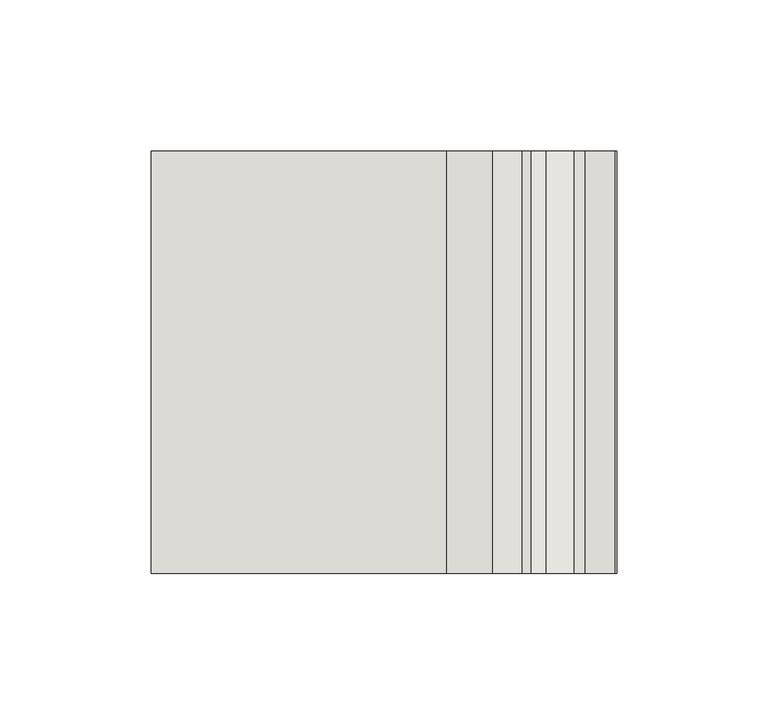
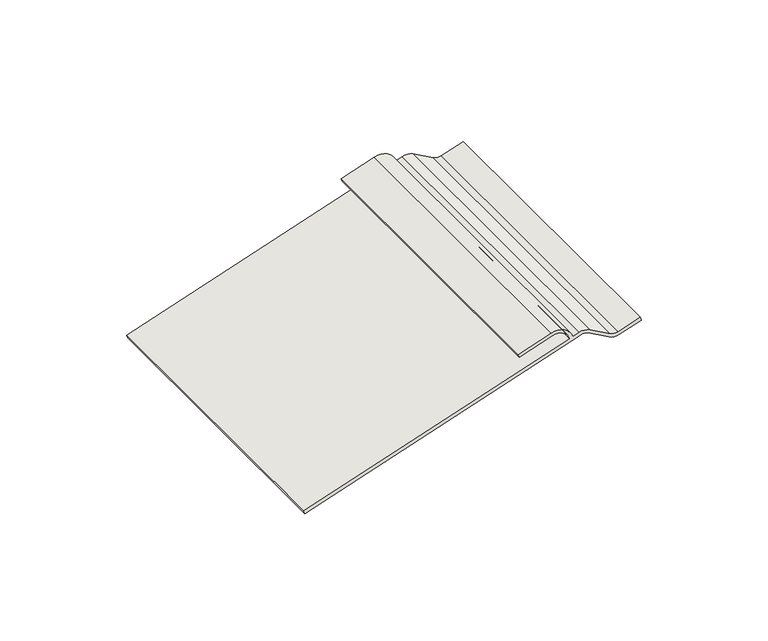
"""IFC4 building model written with IfcOpenShell, lengths in millimetres: wall geometry, BACKUP PLATE : BACKUP PLATE."""

from ifc_helpers import new_model, si_unit, point, frame, frame_2d, origin, place, context, project, spatial, polyline, circle_curve, trimmed, segment, composite_curve, outline, extrude, source, transform, mapped, element, save


def wall_d7630f94(model_context):
    return source(origin(), model_context, "Body", "SweptSolid", [
        extrude(outline(composite_curve([segment(trimmed(circle_curve(frame_2d((5861.775094, 21402.1249746)), 6.28142), [point((5867.3970481, 21404.9267364))], [point((5867.7315606, 21400.1307975))], False, "CARTESIAN"), True, "CONTINUOUS"), segment(polyline([(5867.7315606, 21400.1307975), (5866.7516902, 21397.2039937)]), True, "CONTINUOUS"), segment(trimmed(circle_curve(frame_2d((5864.4121733, 21389.7129802)), 7.8478419), [point((5866.7516902, 21397.2039937))], [point((5871.9007551, 21387.365691))], False, "CARTESIAN"), True, "CONTINUOUS"), segment(polyline([(5871.9007551, 21387.365691), (5866.8391093, 21372.2469118), (5865.3987668, 21372.7291269), (5870.4604125, 21387.8479061)]), True, "CONTINUOUS"), segment(trimmed(circle_curve(frame_2d((5864.3329451, 21389.692997)), 6.3992358), [point((5870.4604125, 21387.8479061))], [point((5866.2781075, 21395.7894354))], True, "CARTESIAN"), True, "CONTINUOUS"), segment(polyline([(5866.2781075, 21395.7894354), (5825.6882747, 21274.5504639), (5824.2479322, 21275.032679), (5866.2912181, 21400.6130126)]), True, "CONTINUOUS"), segment(trimmed(circle_curve(frame_2d((5861.775094, 21402.1249746)), 4.7625), [point((5866.2912181, 21400.6130126))], [point((5866.0375946, 21404.249238))], True, "CARTESIAN"), True, "CONTINUOUS"), segment(polyline([(5866.0375946, 21404.249238), (5860.8088331, 21413.6614781)]), True, "CONTINUOUS"), segment(trimmed(circle_curve(frame_2d((5866.4307872, 21416.4632399)), 6.28142), [point((5860.8088331, 21413.6614781))], [point((5860.4743205, 21418.457417))], False, "CARTESIAN"), True, "CONTINUOUS"), segment(polyline([(5860.4743205, 21418.457417), (5863.8026277, 21428.398836), (5865.2429702, 21427.9166209), (5861.9146631, 21417.9752019)]), True, "CONTINUOUS"), segment(trimmed(circle_curve(frame_2d((5866.4307872, 21416.4632399)), 4.7625), [point((5861.9146631, 21417.9752019))], [point((5862.1682866, 21414.3389765))], True, "CARTESIAN"), True, "CONTINUOUS"), segment(polyline([(5862.1682866, 21414.3389765), (5867.3970481, 21404.9267364)]), True, "CONTINUOUS")], self_intersect=False)), frame((0.0, -1256.0384634, 0.0), z_axis=(0.0, 1.0, 0.0), x_axis=(0.0, 0.0, 1.0)), (0.0, 0.0, 1.0), 139.7),
    ])


if __name__ == "__main__":
    model = new_model("IFC4")
    model_context = context("Model", 3, world=origin())
    ifc_project = project(units=[si_unit("LENGTHUNIT", "METRE", prefix="MILLI")], contexts=[model_context])
    site = spatial("IfcSite", under=ifc_project)
    building = spatial("IfcBuilding", under=site)
    placement = place(None, origin())
    wall_shape = wall_d7630f94(model_context)
    element("IfcWall", 1, ObjectType="BACKUP PLATE : BACKUP PLATE", at=placement, inside=building, context=model_context, shape_type="MappedRepresentation", body=[
        mapped(wall_shape, transform((0.0, 0.0, 0.0), x_axis=(1.0, 0.0, 0.0), y_axis=(0.0, 1.0, 0.0), z_axis=(0.0, 0.0, 1.0))),
    ])
    save(model, "model.ifc")

# Revit data of these elements
# Element 1 (IfcWall, "BACKUP PLATE : BACKUP PLATE")
#   Materials on its faces: "BACKUP PLATE"
# Materials
#   "BACKUP PLATE": class "Generic", colour RGB 195 195 195, transparency 0, Cost = 0
